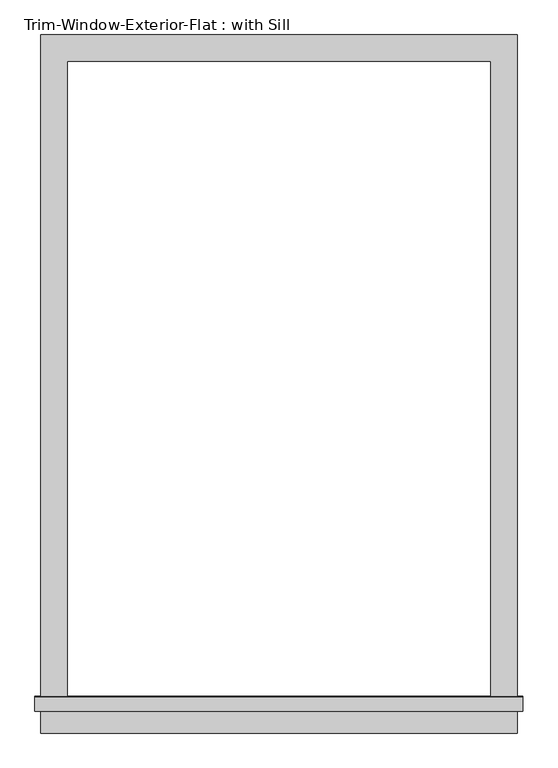
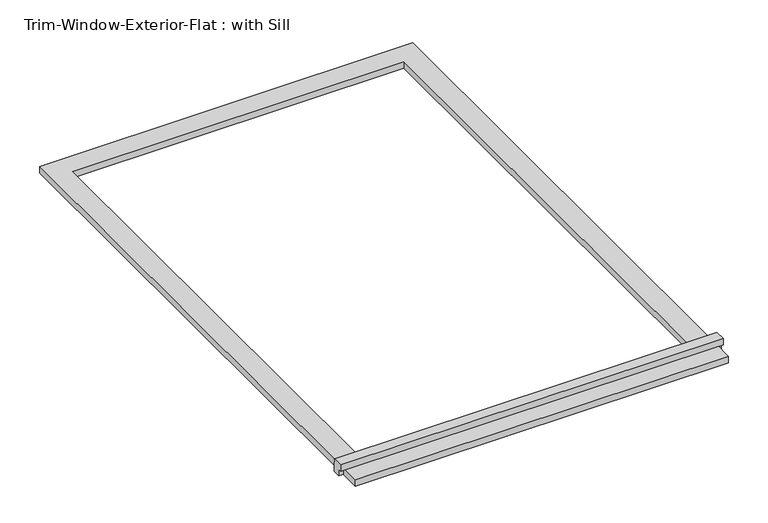
"""IFC4 building model written with IfcOpenShell, lengths in millimetres: proxy geometry, Trim-Window-Exterior-Flat : with Sill."""

import ifcopenshell
import ifcopenshell.guid

model = None  # the IFC model being written
_history = None  # IfcOwnerHistory: only IFC2X3 demands one
_inside = {}  # id of a spatial element -> (the spatial element, [elements in it])
_under = {}  # id of a project, library or spatial element -> (it, [spatial elements below it])
_declared = {}  # id of a project -> (the project, [libraries it declares])
_typed = {}  # id of a type object -> (the type object, [elements of that type])
_made_of = {}  # id of a material, layer set ... -> (it, [elements and type objects made of it])


def new_model(schema):
    """Start an empty IFC model of exactly this schema.

    Asked for "IFC4X3", IfcOpenShell would pick the latest addendum, in which some entities
    have other attributes; the version numbers below select the first issue.
    IFC2X3 requires an IfcOwnerHistory on every rooted entity: one is made here for all.
    """
    global model, _history
    if schema == "IFC4X3":
        model = ifcopenshell.file(schema_version=(4, 3, 0, 0))
    else:
        model = ifcopenshell.file(schema=schema)
    _inside.clear()
    _under.clear()
    _declared.clear()
    _typed.clear()
    _made_of.clear()
    _history = None
    if model.schema == "IFC2X3":
        org = make("IfcOrganization", Name="unknown")
        user = make(
            "IfcPersonAndOrganization",
            ThePerson=make("IfcPerson", FamilyName="unknown"),
            TheOrganization=org,
        )
        app = make(
            "IfcApplication",
            ApplicationDeveloper=org,
            Version="unknown",
            ApplicationFullName="unknown",
            ApplicationIdentifier="unknown",
        )
        _history = make(
            "IfcOwnerHistory",
            OwningUser=user,
            OwningApplication=app,
            ChangeAction="ADDED",
            CreationDate=0,
        )
    return model


def make(cls, **values):
    """One entity of the class cls with the attributes given. An attribute that is None is left unset."""
    return model.create_entity(
        cls, **{name: value for name, value in values.items() if value is not None}
    )


def rooted(cls, **values):
    """An entity with a GlobalId (a new one), such as an element, a storey or a relation."""
    return make(cls, GlobalId=ifcopenshell.guid.new(), OwnerHistory=_history, **values)


def si_unit(unit_type, name, prefix=None):
    """IfcSIUnit, for example si_unit("LENGTHUNIT", "METRE", prefix="MILLI")."""
    return make("IfcSIUnit", UnitType=unit_type, Prefix=prefix, Name=name)


def assignment(units):
    """IfcUnitAssignment: the units of a project."""
    return None if units is None else make("IfcUnitAssignment", Units=units)


def point(xyz):
    """IfcCartesianPoint."""
    return None if xyz is None else make("IfcCartesianPoint", Coordinates=xyz)


def direction(xyz):
    """IfcDirection."""
    return None if xyz is None else make("IfcDirection", DirectionRatios=xyz)


def frame(location, z_axis=None, x_axis=None):
    """IfcAxis2Placement3D, a coordinate frame: its origin and axes. An axis left out is left unset."""
    return make(
        "IfcAxis2Placement3D",
        Location=point(location),
        Axis=direction(z_axis),
        RefDirection=direction(x_axis),
    )


def origin():
    """The frame at (0, 0, 0) with its axes left unset."""
    return frame((0.0, 0.0, 0.0))


def origin_with_axes():
    """The frame at (0, 0, 0) with the z axis (0, 0, 1) and the x axis (1, 0, 0) written out."""
    return frame((0.0, 0.0, 0.0), z_axis=(0.0, 0.0, 1.0), x_axis=(1.0, 0.0, 0.0))


def place(relative_to, where):
    """IfcLocalPlacement: puts the frame where relative to a parent placement (None: the world)."""
    return make(
        "IfcLocalPlacement", PlacementRelTo=relative_to, RelativePlacement=where
    )


def context(
    kind, dimensions, precision=None, world=None, true_north=None, identifier=None
):
    """IfcGeometricRepresentationContext, for example the 3D "Model" context."""
    return make(
        "IfcGeometricRepresentationContext",
        ContextIdentifier=identifier,
        ContextType=kind,
        CoordinateSpaceDimension=dimensions,
        Precision=precision,
        WorldCoordinateSystem=world,
        TrueNorth=true_north,
    )


def project(units=None, contexts=None):
    """IfcProject with its units and contexts."""
    return rooted(
        "IfcProject",
        Name="project",
        RepresentationContexts=contexts,
        UnitsInContext=assignment(units),
    )


def spatial(cls, under=None, at=None, **own):
    """A site, building, storey or space (cls), placed at a placement, below another one or the project."""
    s = rooted(cls, ObjectPlacement=at, **own)
    if under is not None:
        _under.setdefault(under.id(), (under, []))[1].append(s)
    return s


def polyline(points):
    """IfcPolyline through the points."""
    return make("IfcPolyline", Points=[point(p) for p in points])


def outline(outer, holes=None, kind="AREA"):
    """IfcArbitraryClosedProfileDef: a profile drawn as a closed curve; with holes, ...WithVoids."""
    if holes is None:
        return make("IfcArbitraryClosedProfileDef", ProfileType=kind, OuterCurve=outer)
    return make(
        "IfcArbitraryProfileDefWithVoids",
        ProfileType=kind,
        OuterCurve=outer,
        InnerCurves=holes,
    )


def extrude(swept, where, along, depth):
    """IfcExtrudedAreaSolid: the profile swept, set in the frame where, extruded along a direction by depth."""
    return make(
        "IfcExtrudedAreaSolid",
        SweptArea=swept,
        Position=where,
        ExtrudedDirection=direction(along),
        Depth=depth,
    )


def shape(context_of_items, identifier, shape_type, items):
    """IfcShapeRepresentation: the items that make up one representation, for example the "Body"."""
    return make(
        "IfcShapeRepresentation",
        ContextOfItems=context_of_items,
        RepresentationIdentifier=identifier,
        RepresentationType=shape_type,
        Items=items,
    )


def source(mapping_origin, context_of_items, identifier, shape_type, items):
    """IfcRepresentationMap: a shape defined once, which mapped items show again and again."""
    return make(
        "IfcRepresentationMap",
        MappingOrigin=mapping_origin,
        MappedRepresentation=shape(context_of_items, identifier, shape_type, items),
    )


def transform(
    local_origin,
    x_axis=None,
    y_axis=None,
    z_axis=None,
    scale=None,
    scale2=None,
    scale3=None,
    uniform=True,
):
    """IfcCartesianTransformationOperator3D, or its non-uniform kind. x_axis, y_axis, z_axis: its Axis1, 2, 3."""
    if uniform:
        return make(
            "IfcCartesianTransformationOperator3D",
            Axis1=direction(x_axis),
            Axis2=direction(y_axis),
            LocalOrigin=point(local_origin),
            Scale=scale,
            Axis3=direction(z_axis),
        )
    return make(
        "IfcCartesianTransformationOperator3DnonUniform",
        Axis1=direction(x_axis),
        Axis2=direction(y_axis),
        LocalOrigin=point(local_origin),
        Scale=scale,
        Axis3=direction(z_axis),
        Scale2=scale2,
        Scale3=scale3,
    )


def mapped(mapping_source, mapping_target):
    """IfcMappedItem: shows the shape of a source again, moved by a transform."""
    return make(
        "IfcMappedItem", MappingSource=mapping_source, MappingTarget=mapping_target
    )


def made_of(thing, what):
    """Note that an element or type object is made of a material, layer set ...; save() writes the relation."""
    if what is not None:
        _made_of.setdefault(what.id(), (what, []))[1].append(thing)
    return thing


def element(
    cls,
    number,
    at=None,
    inside=None,
    cuts=None,
    type_object=None,
    material=None,
    context=None,
    identifier="Body",
    shape_type=None,
    held_by="IfcProductDefinitionShape",
    body=None,
    shapes=None,
    **own,
):
    """One element of the class cls, such as IfcWall. Its Tag is "e" and its number.

    at: its placement. inside: the storey or other place that contains it. cuts: it is an
    opening in that element (IfcRelVoidsElement). A single representation is given by context,
    identifier, shape_type and body (its items); several are given by shapes. held_by: the class
    of the entity that holds the representations. save() writes the other relations.
    """
    e = rooted(cls, Tag="e%d" % number, ObjectPlacement=at, **own)
    if body is not None:
        shapes = [shape(context, identifier, shape_type, body)]
    if shapes is not None:
        e.Representation = make(held_by, Representations=shapes)
    if inside is not None:
        _inside.setdefault(inside.id(), (inside, []))[1].append(e)
    if cuts is not None:
        rooted(
            "IfcRelVoidsElement", RelatingBuildingElement=cuts, RelatedOpeningElement=e
        )
    if type_object is not None:
        _typed.setdefault(type_object.id(), (type_object, []))[1].append(e)
    return made_of(e, material)


def aggregate(whole, parts):
    """IfcRelAggregates: a whole, such as a stair, and the parts it consists of."""
    return rooted("IfcRelAggregates", RelatingObject=whole, RelatedObjects=parts)


def save(model, path):
    """Write the relations noted so far, then the file.

    IfcRelAggregates (storeys below a building ...), IfcRelContainedInSpatialStructure (elements
    in a storey), IfcRelDefinesByType, IfcRelAssociatesMaterial and IfcRelDeclares: one each for
    every whole, place, type object, material and project.
    """
    for whole, parts in _under.values():
        aggregate(whole, parts)
    for where, things in _inside.values():
        rooted(
            "IfcRelContainedInSpatialStructure",
            RelatedElements=things,
            RelatingStructure=where,
        )
    for kind, things in _typed.values():
        rooted("IfcRelDefinesByType", RelatedObjects=things, RelatingType=kind)
    for what, things in _made_of.values():
        rooted("IfcRelAssociatesMaterial", RelatedObjects=things, RelatingMaterial=what)
    for by, libraries in _declared.values():
        rooted("IfcRelDeclares", RelatingContext=by, RelatedDefinitions=libraries)
    model.write(path)


def trim_window_exterior_flat_with_sill_8899ae9c(model_context):
    return source(origin(), model_context, "Body", "SweptSolid", [
        extrude(outline(polyline([(514.35, -1393.7823709), (514.35, -1450.9323709), (-514.35, -1450.9323709), (-514.35, -1393.7823709), (514.35, -1393.7823709)])), origin_with_axes(), (0.0, 0.0, 1.0), 19.05),
        extrude(outline(polyline([(-1403.35, 38.1), (-1374.0580645, 38.1), (-1371.6, 19.05), (-1371.6, 0.0), (-1393.7823709, 0.0), (-1393.7823709, 19.05), (-1403.35, 19.05), (-1403.35, 38.1)])), frame((-527.05, 0.0, 0.0), z_axis=(1.0, 0.0, 0.0), x_axis=(0.0, 1.0, 0.0)), (0.0, 0.0, 1.0), 1054.1),
        extrude(outline(polyline([(-514.35, 57.15), (514.35, 57.15), (514.35, -1371.6), (457.2, -1371.6), (457.2, 0.0), (-457.2, 0.0), (-457.2, -1371.6), (-514.35, -1371.6), (-514.35, 57.15)])), origin_with_axes(), (0.0, 0.0, 1.0), 19.05),
    ])


if __name__ == "__main__":
    model = new_model("IFC4")
    model_context = context("Model", 3, world=origin())
    ifc_project = project(units=[si_unit("LENGTHUNIT", "METRE", prefix="MILLI")], contexts=[model_context])
    site = spatial("IfcSite", under=ifc_project)
    building = spatial("IfcBuilding", under=site)
    placement = place(None, origin())
    trim_window_exterior_flat_with_sill_shape = trim_window_exterior_flat_with_sill_8899ae9c(model_context)
    element("IfcBuildingElementProxy", 1, Name="Trim-Window-Exterior-Flat : with Sill", ObjectType="Trim-Window-Exterior-Flat : with Sill", at=placement, inside=building, context=model_context, shape_type="MappedRepresentation", body=[
        mapped(trim_window_exterior_flat_with_sill_shape, transform((0.0, 0.0, 0.0), x_axis=(1.0, 0.0, 0.0), y_axis=(0.0, 1.0, 0.0), z_axis=(0.0, 0.0, 1.0))),
    ])
    save(model, "model.ifc")

# Revit data of these elements
# Type "Trim-Window-Exterior-Flat : with Sill"
#   Trim Width = 0' - 2 1/4"
#   Trim Thickness_Picture Frame = 0' - 1 1/4"
#   Trim Thickness_with Sill = 0' - 0 3/4"
#   Sill Thickness = 0' - 1 1/4"
#   Opening Width [instance default] = 2' - 0"
#   Opening Height [instance default] = 3' - 0"
#   Default Elevation = 4' - 0"
#   Sill = yes
#   Picture Frame = no
#   Trim Material [instance default] = none
# Element 1 (IfcBuildingElementProxy, "Trim-Window-Exterior-Flat : with Sill")
#   Opening Width = 3' - 0"
#   Opening Height = 4' - 6"
#   Trim Material = Clad - White
#   Materials on its faces: "Clad - White"
# Materials
#   "Clad - White": class "Wood", colour RGB 242 242 238, transparency 0, Cost = 0
